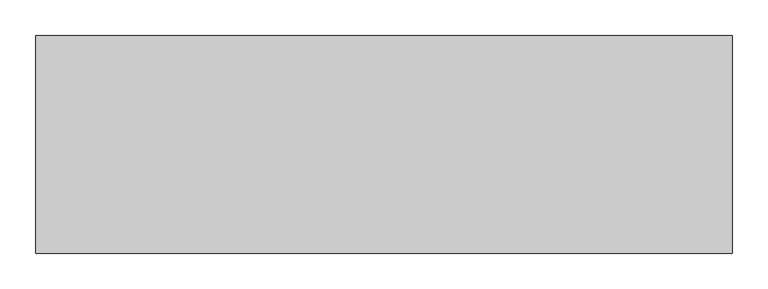
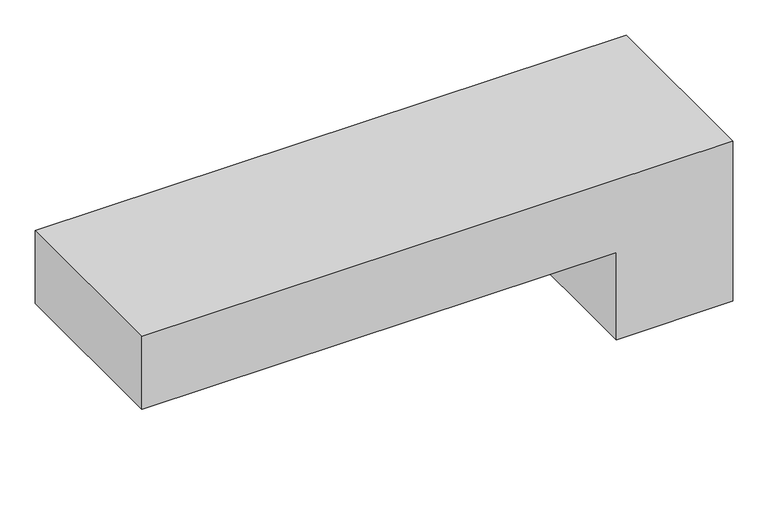
"""IFC4 building model written with IfcOpenShell, lengths in millimetres: proxy geometry, Generic Models 290:Generic Models 290:154933 : Generic Models 290:Generic Models 290:154933."""

from ifc_helpers import new_model, si_unit, frame, origin, place, context, project, spatial, polyline, outline, extrude, source, transform, mapped, element, save


def generic_models_05fdad31(model_context):
    return source(origin(), model_context, "Body", "SweptSolid", [
        extrude(outline(polyline([(-152.4, 6829.303213), (127.0, 6829.303213), (127.0, 5854.4339355), (0.0, 5854.4339355), (0.0, 6636.705853), (-152.4, 6636.705853), (-152.4, 6829.303213)])), frame((0.0, 8404.9928291, 0.0), z_axis=(0.0, 1.0, 0.0), x_axis=(0.0, 0.0, 1.0)), (0.0, 0.0, 1.0), 304.8),
    ])


if __name__ == "__main__":
    model = new_model("IFC4")
    model_context = context("Model", 3, world=origin())
    ifc_project = project(units=[si_unit("LENGTHUNIT", "METRE", prefix="MILLI")], contexts=[model_context])
    site = spatial("IfcSite", under=ifc_project)
    building = spatial("IfcBuilding", under=site)
    placement = place(None, origin())
    generic_models_shape = generic_models_05fdad31(model_context)
    element("IfcBuildingElementProxy", 1, Name="Generic Models 290:Generic Models 290:154933 : Generic Models 290:Generic Models 290:154933", ObjectType="Generic Models 290:Generic Models 290:154933 : Generic Models 290:Generic Models 290:154933", at=placement, inside=building, context=model_context, shape_type="MappedRepresentation", body=[
        mapped(generic_models_shape, transform((0.0, 0.0, 0.0), x_axis=(1.0, 0.0, 0.0), y_axis=(0.0, 1.0, 0.0), z_axis=(0.0, 0.0, 1.0))),
    ])
    save(model, "model.ifc")

# Revit data of these elements
# Type "Generic Models 290:Generic Models 290:154933 : Generic Models 290:Generic Models 290:154933"
#   NameOverride = "Generic Models 290:Generic Models 290:154933"
#   ObjectTypeOverride = "Generic Models 290:Generic Models 290"
#   Reference = "Generic Models 290"
#   Category = "Generic Models"
#   Tag = "154933"
# Element 1 (IfcBuildingElementProxy, "Generic Models 290:Generic Models 290:154933 : Generic Models 290:Generic Models 290:154933")
#   Materials on its faces: "_ 8\" CONCRETE SLAB W/ GRADE BEAM (SEE STRUCT. DWGS) 10051"
# Materials
#   "_ 8\" CONCRETE SLAB W/ GRADE BEAM (SEE STRUCT. DWGS) 10051": class "Unassigned", colour RGB 191 191 191, transparency 0
